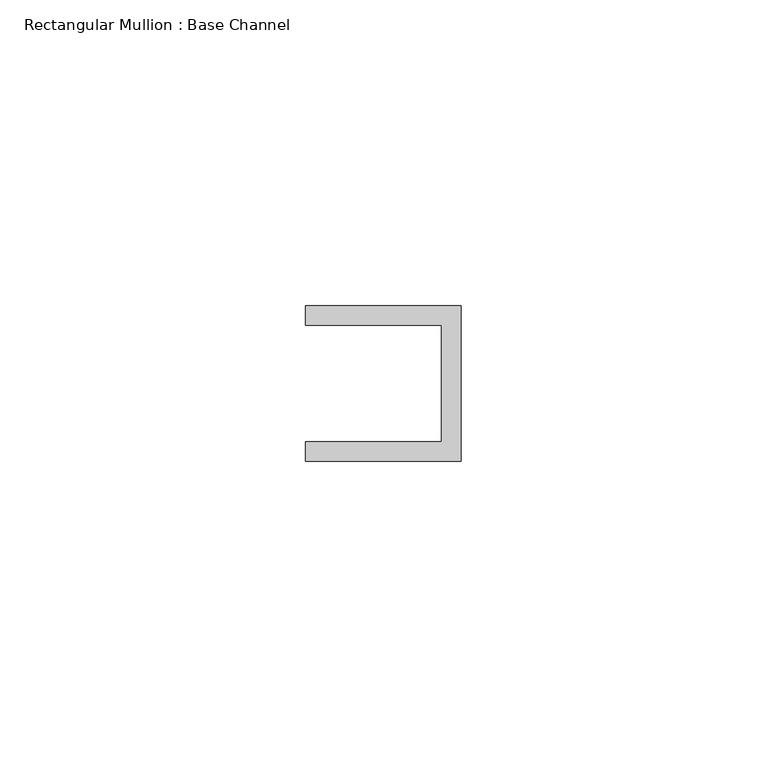
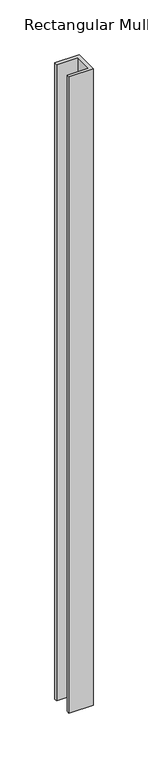
"""IFC4 building model written with IfcOpenShell, lengths in millimetres: member geometry, Rectangular Mullion : Base Channel."""

from ifc_helpers import new_model, si_unit, frame, origin, place, context, project, spatial, polyline, outline, extrude, source, transform, mapped, element, save


def rectangular_mullion_base_channel_8e9ccb36(model_context):
    return source(origin(), model_context, "Body", "SweptSolid", [
        extrude(outline(polyline([(0.0, -12.7), (-25.4, -12.7), (-25.4, -9.525), (-3.175, -9.525), (-3.175, 9.525), (-25.4, 9.525), (-25.4, 12.7), (0.0, 12.7), (0.0, -12.7)])), frame((0.0, 0.0, -706.9666667), z_axis=(0.0, 0.0, 1.0), x_axis=(1.0, 0.0, 0.0)), (0.0, 0.0, 1.0), 706.9666667),
    ])


if __name__ == "__main__":
    model = new_model("IFC4")
    model_context = context("Model", 3, world=origin())
    ifc_project = project(units=[si_unit("LENGTHUNIT", "METRE", prefix="MILLI")], contexts=[model_context])
    site = spatial("IfcSite", under=ifc_project)
    building = spatial("IfcBuilding", under=site)
    placement = place(None, origin())
    rectangular_mullion_base_channel_shape = rectangular_mullion_base_channel_8e9ccb36(model_context)
    element("IfcMember", 1, ObjectType="Rectangular Mullion : Base Channel", at=placement, inside=building, context=model_context, shape_type="MappedRepresentation", body=[
        mapped(rectangular_mullion_base_channel_shape, transform((0.0, 0.0, 0.0), x_axis=(1.0, 0.0, 0.0), y_axis=(0.0, 1.0, 0.0), z_axis=(0.0, 0.0, 1.0))),
    ])
    save(model, "model.ifc")

# Revit data of these elements
# Type "Rectangular Mullion : Base Channel"
#   built-in parameter 1007322 = 0.0833333 (stored number, unit not read)
#   built-in parameter 1007321 = 0.0416667 (stored number, unit not read)
#   built-in parameter 1007320 = -0.03125 (stored number, unit not read)
# Element 1 (IfcMember, "Rectangular Mullion : Base Channel")
#   Materials on its faces: "ALUM"
# Materials
#   "ALUM": class "Generic", colour RGB 157 157 157, transparency 0, Cost = 0
